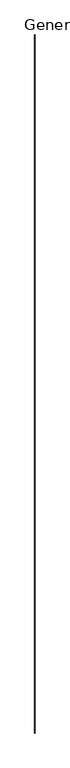
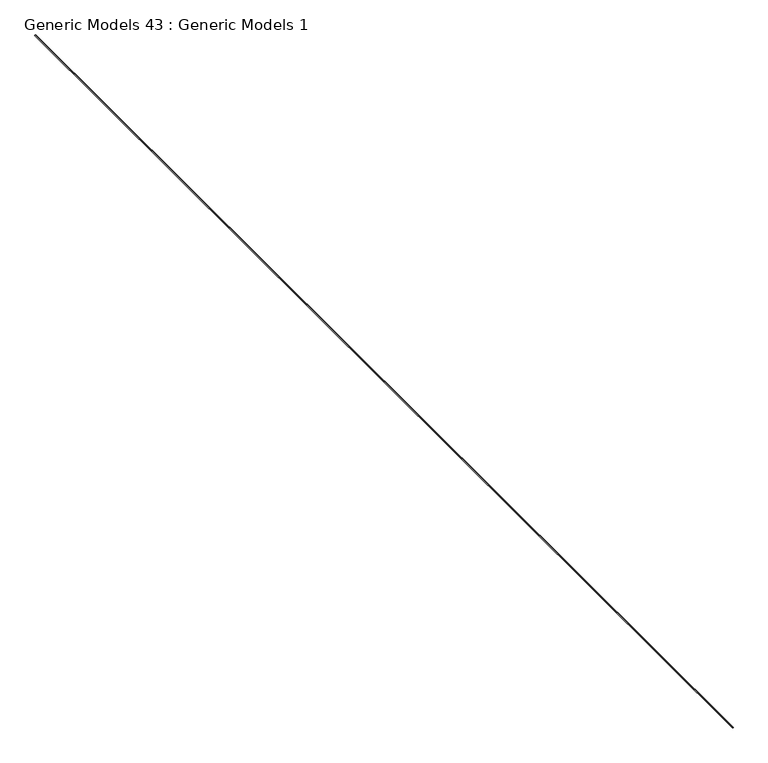
"""IFC4 building model written with IfcOpenShell, lengths in millimetres: proxy geometry, Generic Models 43 : Generic Models 1."""

from ifc_helpers import new_model, si_unit, point, frame, origin, place, context, project, spatial, polyline, circle_curve, ellipse_curve, trimmed, source, transform, mapped, element, save
from ifc_brep_helpers import plane_surface, cylinder_surface, revolved_surface, extruded_surface, advanced_brep


def generic_models_43_generic_models_1_61a04976(model_context):
    return source(origin(), model_context, "Body", "AdvancedBrep", [
        advanced_brep(
        [(32147.5090778, 25672.1156612, 268893.925), (32144.3340778, 25672.1156612, 268893.925), (32143.3823185, 25672.1156612, 268892.6543414), (32143.3823185, 25672.1156612, 268888.8456586), (32144.3340778, 25672.1156612, 268887.575), (32147.5090778, 25672.1156612, 268887.575), (32147.5090778, 40827.6606612, 268893.925), (32147.5090778, 40827.6606612, 268887.575), (32144.3340778, 40827.6606612, 268887.575), (32143.3823185, 40827.6606612, 268888.8456586), (32143.3823185, 40827.6606612, 268892.6543414), (32144.3340778, 40827.6606612, 268893.925)],
        [
            (0, 1),
            (1, 2, circle_curve(frame((32147.2488183, 25672.1156612, 268890.75), z_axis=(0.0, -1.0, 0.0), x_axis=(0.0, 0.0, 1.0)), 4.3100275)),
            (2, 3, ellipse_curve(frame((32139.5715778, 25672.1156612, 268890.75), z_axis=(0.0, -1.0, 0.0), x_axis=(1.0, 0.0, 0.0)), 4.7625, 3.175)),
            (3, 4, circle_curve(frame((32147.2488183, 25672.1156612, 268890.75), z_axis=(0.0, -1.0, 0.0), x_axis=(0.0, 0.0, 1.0)), 4.3100275)),
            (4, 5),
            (5, 0, circle_curve(frame((32150.4238183, 25672.1156612, 268890.75), z_axis=(0.0, 1.0, 0.0), x_axis=(0.0, 0.0, 1.0)), 4.3100275)),
            (6, 7, circle_curve(frame((32150.4238183, 40827.6606612, 268890.75), z_axis=(0.0, -1.0, 0.0), x_axis=(0.0, 0.0, 1.0)), 4.3100275)),
            (7, 8),
            (8, 9, circle_curve(frame((32147.2488183, 40827.6606612, 268890.75), z_axis=(0.0, 1.0, 0.0), x_axis=(0.0, 0.0, 1.0)), 4.3100275)),
            (9, 10, ellipse_curve(frame((32139.5715778, 40827.6606612, 268890.75), z_axis=(0.0, 1.0, 0.0), x_axis=(1.0, 0.0, 0.0)), 4.7625, 3.175)),
            (10, 11, circle_curve(frame((32147.2488183, 40827.6606612, 268890.75), z_axis=(0.0, 1.0, 0.0), x_axis=(0.0, 0.0, 1.0)), 4.3100275)),
            (11, 6),
            (5, 7),
            (6, 0),
            (11, 1),
            (3, 9),
            (8, 4),
            (2, 10),
        ],
        [
            plane_surface(frame((32147.5090778, 25672.1156612, 268887.575), z_axis=(0.0, -1.0, 0.0), x_axis=(0.0, 0.0, 1.0))),
            plane_surface(frame((32147.5090778, 40827.6606612, 268887.575), z_axis=(0.0, 1.0, 0.0), x_axis=(0.0, 0.0, 1.0))),
            revolved_surface(polyline([(32150.4238183, 40827.6606612, 268895.0600275), (32150.4238183, 25672.1156612, 268895.0600275)]), (32150.4238183, 25672.1156612, 268890.75), (0.0, 1.0, 0.0)),
            plane_surface(frame((32147.5090778, 25672.1156612, 268893.925), z_axis=(0.0, 0.0, 1.0), x_axis=(0.0, 1.0, 0.0))),
            cylinder_surface(frame((32147.2488183, 25672.1156612, 268890.75), z_axis=(0.0, -1.0, 0.0), x_axis=(0.0, 0.0, 1.0)), 4.3100275),
            plane_surface(frame((32144.3340778, 25672.1156612, 268887.575), z_axis=(0.0, 0.0, -1.0), x_axis=(0.0, 1.0, 0.0))),
            extruded_surface(trimmed(ellipse_curve(frame((32139.5715778, 40827.6606612, 268890.75), z_axis=(0.0, -1.0, 0.0), x_axis=(1.0, 0.0, 0.0)), 4.7625, 3.175), [point((32143.3823185, 40827.6606612, 268892.6543414))], [point((32143.3823185, 40827.6606612, 268888.8456586))], True, "CARTESIAN"), (0.0, -15155.545000000002, 0.0), 15155.545000000002),
        ],
        [
            (0, [[1, 2, 3, 4, 5, 6]]),
            (1, [[7, 8, 9, 10, 11, 12]]),
            (2, [[-6, 13, -7, 14]]),
            (3, [[-1, -14, -12, 15]]),
            (4, [[-4, 16, -9, 17]]),
            (5, [[-5, -17, -8, -13]]),
            (6, [[-3, 18, -10, -16]]),
            (4, [[-2, -15, -11, -18]]),
        ],
    ),
    ])


if __name__ == "__main__":
    model = new_model("IFC4")
    model_context = context("Model", 3, world=origin())
    ifc_project = project(units=[si_unit("LENGTHUNIT", "METRE", prefix="MILLI")], contexts=[model_context])
    site = spatial("IfcSite", under=ifc_project)
    building = spatial("IfcBuilding", under=site)
    placement = place(None, origin())
    generic_models_43_generic_models_1_shape = generic_models_43_generic_models_1_61a04976(model_context)
    element("IfcBuildingElementProxy", 1, Name="Generic Models 43 : Generic Models 1", ObjectType="Generic Models 43 : Generic Models 1", at=placement, inside=building, context=model_context, shape_type="MappedRepresentation", body=[
        mapped(generic_models_43_generic_models_1_shape, transform((0.0, 0.0, 0.0), x_axis=(1.0, 0.0, 0.0), y_axis=(0.0, 1.0, 0.0), z_axis=(0.0, 0.0, 1.0))),
    ])
    save(model, "model.ifc")

# Revit data of these elements
# Element 1 (IfcBuildingElementProxy, "Generic Models 43 : Generic Models 1")
#   Materials on its faces: "SEALANT (& BACKER ROD IF NECESSARY)"
# Materials
#   "SEALANT (& BACKER ROD IF NECESSARY)": class "Generic", colour RGB 176 213 108, transparency 0, Cost = 0
